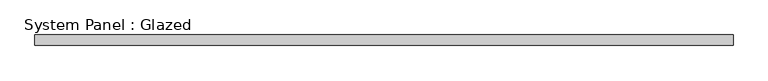
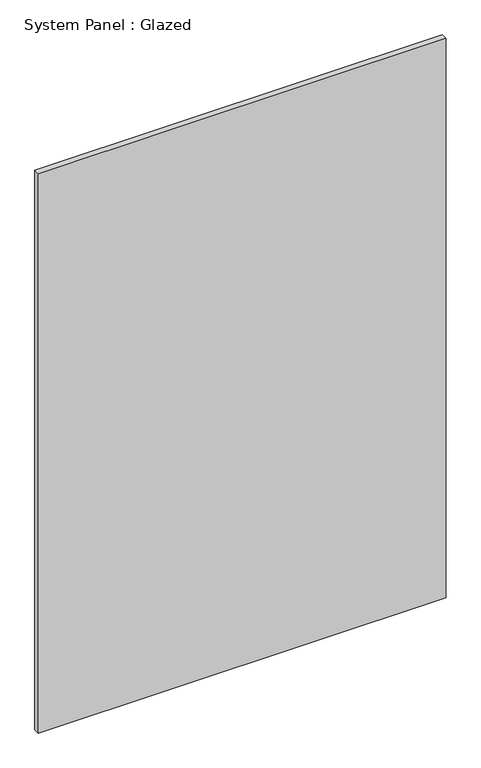
"""IFC4 building model written with IfcOpenShell, lengths in millimetres: plate geometry, System Panel : Glazed."""

from ifc_helpers import new_model, si_unit, origin, origin_with_axes, place, context, project, spatial, polyline, outline, extrude, source, transform, mapped, element, save


def system_panel_glazed_0b996a41(model_context):
    return source(origin(), model_context, "Body", "SweptSolid", [
        extrude(outline(polyline([(827.5000002, 24.5), (-827.5000002, 24.5), (-827.5000002, 49.5), (827.5000002, 49.5), (827.5000002, 24.5)])), origin_with_axes(), (0.0, 0.0, 1.0), 2400.0),
    ])


if __name__ == "__main__":
    model = new_model("IFC4")
    model_context = context("Model", 3, world=origin())
    ifc_project = project(units=[si_unit("LENGTHUNIT", "METRE", prefix="MILLI")], contexts=[model_context])
    site = spatial("IfcSite", under=ifc_project)
    building = spatial("IfcBuilding", under=site)
    placement = place(None, origin())
    system_panel_glazed_shape = system_panel_glazed_0b996a41(model_context)
    element("IfcPlate", 1, ObjectType="System Panel : Glazed", at=placement, inside=building, context=model_context, shape_type="MappedRepresentation", body=[
        mapped(system_panel_glazed_shape, transform((0.0, 0.0, 0.0), x_axis=(1.0, 0.0, 0.0), y_axis=(0.0, 1.0, 0.0), z_axis=(0.0, 0.0, 1.0))),
    ])
    save(model, "model.ifc")

# Revit data of these elements
# Type "System Panel : Glazed"
#   Keynote = "H11"
#   Construction Type Id = "GSP4R"
#   Analytic Construction = "1/8 in Pilkington single glazing"
#   Visual Light Transmittance = 0.9
#   Solar Heat Gain Coefficient = 0.86
#   Heat Transfer Coefficient (U) = 6.7069 W/(m²·K)
#   Define Thermal Properties by = 1
# Element 1 (IfcPlate, "System Panel : Glazed")
#   Materials on its faces: "Glass"
# Materials
#   "Glass": class "Glass", colour RGB 0 128 192, transparency 0.9, Description = "Soda Lime Glass", Cost = 0
